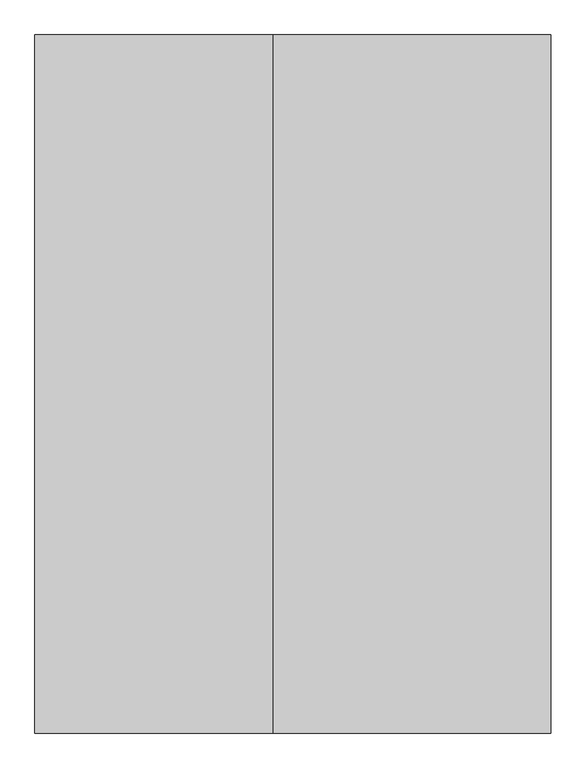
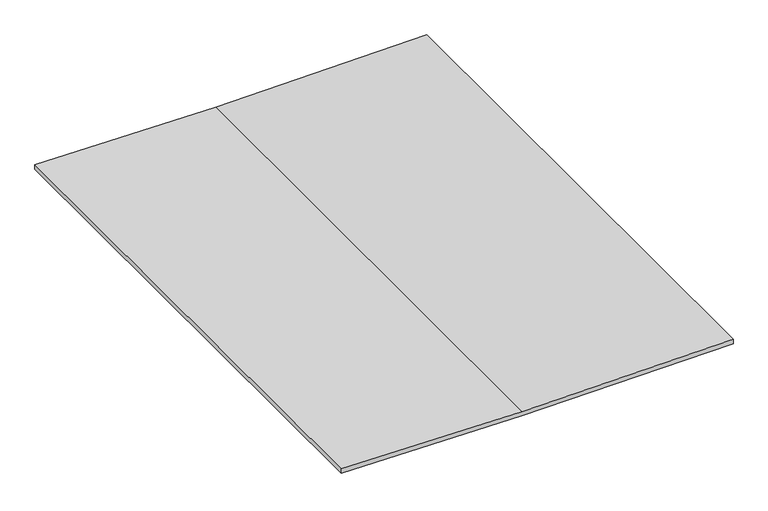
"""IFC4 building model written with IfcOpenShell, lengths in millimetres: proxy geometry, COVER BOARD002 14707 : COVER BOARD002 14707."""

from ifc_helpers import new_model, si_unit, frame, origin, place, context, project, spatial, polyline, outline, extrude, source, transform, mapped, element, save


def generic_models_e83da0d9(model_context):
    return source(origin(), model_context, "Body", "SweptSolid", [
        extrude(outline(polyline([(40228.1021556, -1886.5629484), (40237.9000089, -2567.3737014), (40220.5682898, -2567.3737014), (40210.7704365, -1886.5629484), (40220.5682898, -1090.0815411), (40237.9000089, -1090.0815411), (40228.1021556, -1886.5629484)])), frame((0.0, 1000.0, 0.0), z_axis=(0.0, 1.0, 0.0), x_axis=(0.0, 0.0, 1.0)), (0.0, 0.0, 1.0), 2000.0),
    ])


if __name__ == "__main__":
    model = new_model("IFC4")
    model_context = context("Model", 3, world=origin())
    ifc_project = project(units=[si_unit("LENGTHUNIT", "METRE", prefix="MILLI")], contexts=[model_context])
    site = spatial("IfcSite", under=ifc_project)
    building = spatial("IfcBuilding", under=site)
    placement = place(None, origin())
    generic_models_shape = generic_models_e83da0d9(model_context)
    element("IfcBuildingElementProxy", 1, Name="COVER BOARD002 14707 : COVER BOARD002 14707", ObjectType="COVER BOARD002 14707 : COVER BOARD002 14707", at=placement, inside=building, context=model_context, shape_type="MappedRepresentation", body=[
        mapped(generic_models_shape, transform((0.0, 0.0, 0.0), x_axis=(1.0, 0.0, 0.0), y_axis=(0.0, 1.0, 0.0), z_axis=(0.0, 0.0, 1.0))),
    ])
    save(model, "model.ifc")

# Revit data of these elements
# Type "COVER BOARD002 14707 : COVER BOARD002 14707"
#   NameOverride = "COVER BOARD002"
# Element 1 (IfcBuildingElementProxy, "COVER BOARD002 14707 : COVER BOARD002 14707")
#   Materials on its faces: "CDX PLYWOOD - SEE STRUCTURAL DWGS"
# Materials
#   "CDX PLYWOOD - SEE STRUCTURAL DWGS": class "Unassigned", colour RGB 138 93 50, transparency 0, Cost = 0
